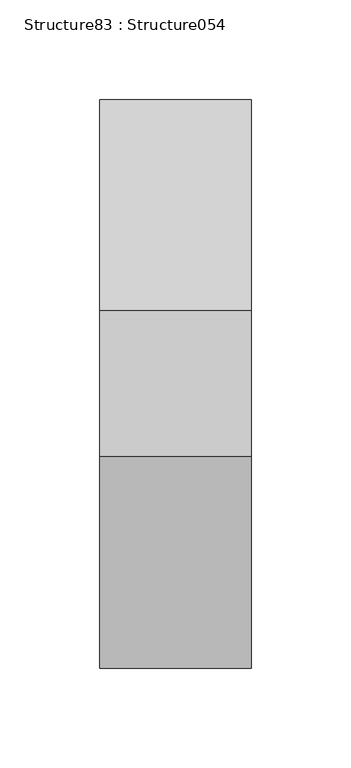
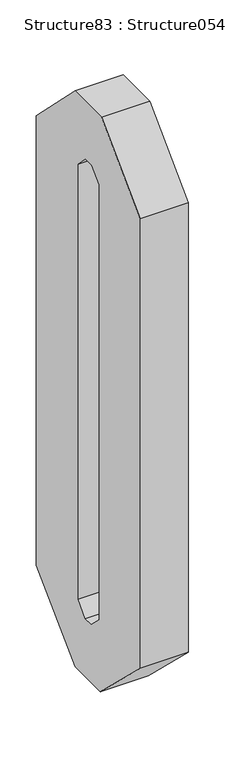
"""IFC4 building model written with IfcOpenShell, lengths in millimetres: proxy geometry, Structure83 : Structure054."""

from ifc_helpers import new_model, si_unit, frame, origin, place, context, project, spatial, polyline, outline, extrude, source, transform, mapped, element, save


def structure83_structure054_0ae66cba(model_context):
    return source(origin(), model_context, "Body", "SweptSolid", [
        extrude(outline(polyline([(284419.3729591, 4382.5453733), (284419.3729591, 3629.2077294), (284313.3070282, 3523.1417985), (284243.8122141, 3523.2149577), (284133.8087542, 3629.2065158), (284133.8074946, 4382.5456393), (284239.8734256, 4488.6115703), (284313.3070282, 4488.6115703), (284419.3729591, 4382.5453733)]), holes=[polyline([(284268.4310426, 3621.0476006), (284284.7456324, 3621.0482303), (284305.1437503, 3641.4463659), (284305.1437503, 4370.299463), (284284.7456324, 4390.697581), (284268.4304129, 4390.697581), (284248.0322949, 4370.299463), (284248.0322949, 3641.4461544), (284268.4310426, 3621.0476006)])]), frame((-59031.6926606, 0.0, 0.0), z_axis=(1.0, 0.0, 0.0), x_axis=(0.0, 1.0, 0.0)), (0.0, 0.0, 1.0), 76.2),
    ])


if __name__ == "__main__":
    model = new_model("IFC4")
    model_context = context("Model", 3, world=origin())
    ifc_project = project(units=[si_unit("LENGTHUNIT", "METRE", prefix="MILLI")], contexts=[model_context])
    site = spatial("IfcSite", under=ifc_project)
    building = spatial("IfcBuilding", under=site)
    placement = place(None, origin())
    structure83_structure054_shape = structure83_structure054_0ae66cba(model_context)
    element("IfcBuildingElementProxy", 1, Name="Structure83 : Structure054", ObjectType="Structure83 : Structure054", at=placement, inside=building, context=model_context, shape_type="MappedRepresentation", body=[
        mapped(structure83_structure054_shape, transform((0.0, 0.0, 0.0), x_axis=(1.0, 0.0, 0.0), y_axis=(0.0, 1.0, 0.0), z_axis=(0.0, 0.0, 1.0))),
    ])
    save(model, "model.ifc")

# Revit data of these elements
# Type "Structure83 : Structure054"
#   NameOverride = "Structure054"
# Element 1 (IfcBuildingElementProxy, "Structure83 : Structure054")
#   Materials on its faces: "BRUSHED ALUM. LETTERING"
# Materials
#   "BRUSHED ALUM. LETTERING": class "Unassigned", colour RGB 169 181 186, transparency 0, Cost = 0
